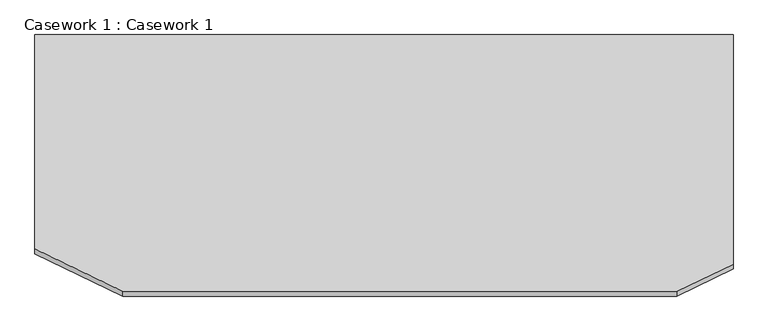
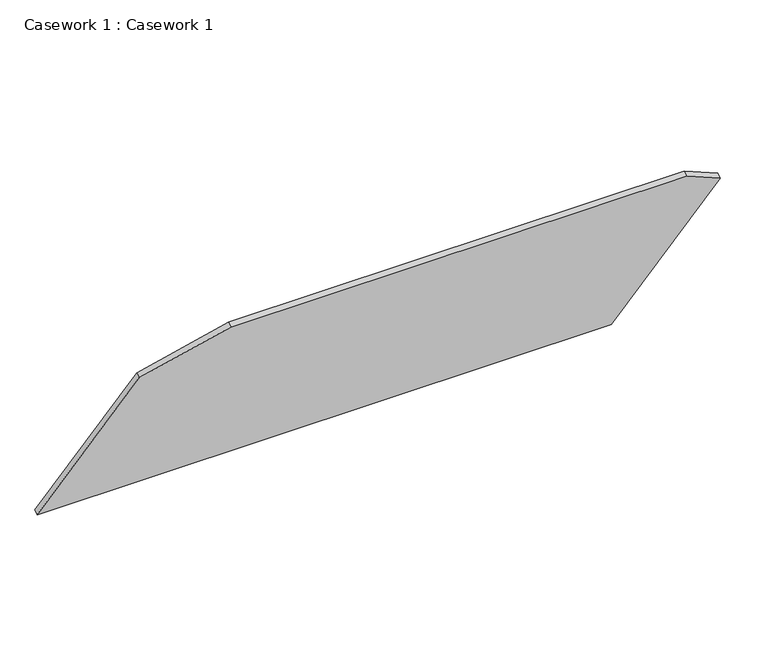
"""IFC4 building model written with IfcOpenShell, lengths in millimetres: furniture geometry, Casework 1 : Casework 1."""

from ifc_helpers import new_model, si_unit, frame, origin, place, context, project, spatial, polyline, outline, extrude, source, transform, mapped, element, save


def casework_1_casework_1_270aac2f(model_context):
    return source(origin(), model_context, "Body", "SweptSolid", [
        extrude(outline(polyline([(-386.9754356, 0.0), (974.7148655, 0.0), (1135.9371116, -192.1371911), (1135.9371116, -2076.38239), (885.3671852, -2375.0), (-386.9754356, -2375.0), (-386.9754356, 0.0)])), frame((-5120.0247381, 1566.782226, 5553.4812607), z_axis=(0.0, 0.8191520442889929, 0.5735764363510446), x_axis=(0.0, -0.5735764363510446, 0.8191520442889929)), (0.0, 0.0, 1.0), 20.0),
    ])


if __name__ == "__main__":
    model = new_model("IFC4")
    model_context = context("Model", 3, world=origin())
    ifc_project = project(units=[si_unit("LENGTHUNIT", "METRE", prefix="MILLI")], contexts=[model_context])
    site = spatial("IfcSite", under=ifc_project)
    building = spatial("IfcBuilding", under=site)
    placement = place(None, origin())
    casework_1_casework_1_shape = casework_1_casework_1_270aac2f(model_context)
    element("IfcFurniture", 1, ObjectType="Casework 1 : Casework 1", at=placement, inside=building, context=model_context, shape_type="MappedRepresentation", body=[
        mapped(casework_1_casework_1_shape, transform((0.0, 0.0, 0.0), x_axis=(1.0, 0.0, 0.0), y_axis=(0.0, 1.0, 0.0), z_axis=(0.0, 0.0, 1.0))),
    ])
    save(model, "model.ifc")

# Revit data of these elements
# Element 1 (IfcFurniture, "Casework 1 : Casework 1")
#   Materials on its faces: "Plaster"
# Materials
#   "Plaster": class "Generic", colour RGB 249 249 249, transparency 0, Description = "Plaster", Cost = 0
